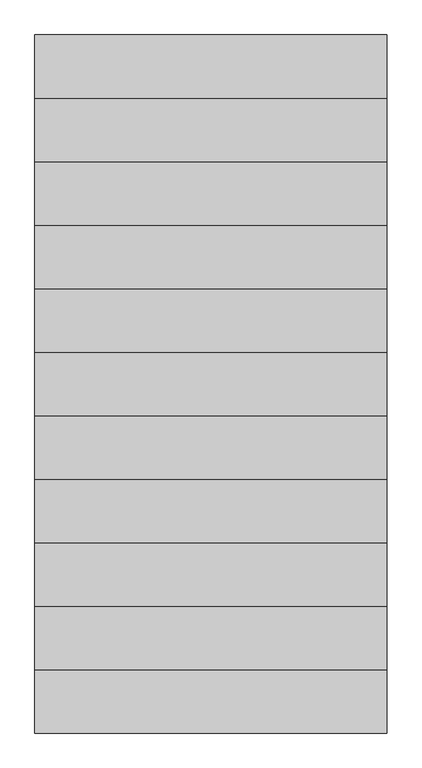
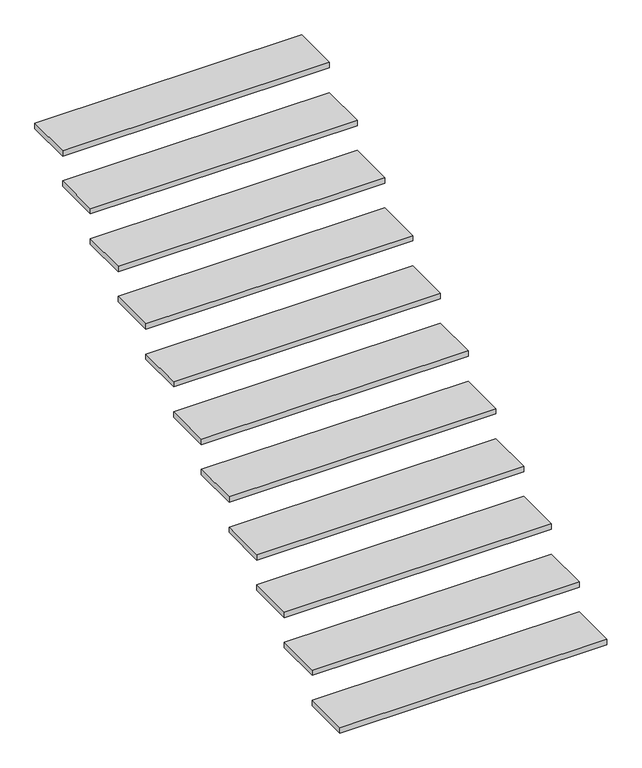
"""IFC4 building model written with IfcOpenShell, lengths in millimetres: stair flight geometry."""

from ifc_helpers import new_model, si_unit, frame, origin, place, context, project, spatial, polyline, outline, extrude, source, transform, mapped, element, save


def stair_flight_466a32d1(model_context):
    return source(origin(), model_context, "Body", "SweptSolid", [
        extrude(outline(polyline([(17005.3403387, 2217.6066446), (18505.3403387, 2217.6066446), (18505.3403387, 1947.6066446), (17005.3403387, 1947.6066446), (17005.3403387, 2217.6066446)])), frame((0.0, 0.0, 11969.0989011), z_axis=(0.0, 0.0, 1.0), x_axis=(1.0, 0.0, 0.0)), (0.0, 0.0, 1.0), 32.0),
        extrude(outline(polyline([(17005.3403387, 2487.6066446), (18505.3403387, 2487.6066446), (18505.3403387, 2217.6066446), (17005.3403387, 2217.6066446), (17005.3403387, 2487.6066446)])), frame((0.0, 0.0, 12148.2197802), z_axis=(0.0, 0.0, 1.0), x_axis=(1.0, 0.0, 0.0)), (0.0, 0.0, 1.0), 32.0),
        extrude(outline(polyline([(17005.3403387, 2757.6066446), (18505.3403387, 2757.6066446), (18505.3403387, 2487.6066446), (17005.3403387, 2487.6066446), (17005.3403387, 2757.6066446)])), frame((0.0, 0.0, 12327.3406593), z_axis=(0.0, 0.0, 1.0), x_axis=(1.0, 0.0, 0.0)), (0.0, 0.0, 1.0), 32.0),
        extrude(outline(polyline([(17005.3403387, 3027.6066446), (18505.3403387, 3027.6066446), (18505.3403387, 2757.6066446), (17005.3403387, 2757.6066446), (17005.3403387, 3027.6066446)])), frame((0.0, 0.0, 12506.4615385), z_axis=(0.0, 0.0, 1.0), x_axis=(1.0, 0.0, 0.0)), (0.0, 0.0, 1.0), 32.0),
        extrude(outline(polyline([(17005.3403387, 3297.6066446), (18505.3403387, 3297.6066446), (18505.3403387, 3027.6066446), (17005.3403387, 3027.6066446), (17005.3403387, 3297.6066446)])), frame((0.0, 0.0, 12685.5824176), z_axis=(0.0, 0.0, 1.0), x_axis=(1.0, 0.0, 0.0)), (0.0, 0.0, 1.0), 32.0),
        extrude(outline(polyline([(17005.3403387, 3567.6066446), (18505.3403387, 3567.6066446), (18505.3403387, 3297.6066446), (17005.3403387, 3297.6066446), (17005.3403387, 3567.6066446)])), frame((0.0, 0.0, 12864.7032967), z_axis=(0.0, 0.0, 1.0), x_axis=(1.0, 0.0, 0.0)), (0.0, 0.0, 1.0), 32.0),
        extrude(outline(polyline([(17005.3403387, 3837.6066446), (18505.3403387, 3837.6066446), (18505.3403387, 3567.6066446), (17005.3403387, 3567.6066446), (17005.3403387, 3837.6066446)])), frame((0.0, 0.0, 13043.8241758), z_axis=(0.0, 0.0, 1.0), x_axis=(1.0, 0.0, 0.0)), (0.0, 0.0, 1.0), 32.0),
        extrude(outline(polyline([(17005.3403387, 4107.6066446), (18505.3403387, 4107.6066446), (18505.3403387, 3837.6066446), (17005.3403387, 3837.6066446), (17005.3403387, 4107.6066446)])), frame((0.0, 0.0, 13222.9450549), z_axis=(0.0, 0.0, 1.0), x_axis=(1.0, 0.0, 0.0)), (0.0, 0.0, 1.0), 32.0),
        extrude(outline(polyline([(17005.3403387, 4377.6066446), (18505.3403387, 4377.6066446), (18505.3403387, 4107.6066446), (17005.3403387, 4107.6066446), (17005.3403387, 4377.6066446)])), frame((0.0, 0.0, 13402.0659341), z_axis=(0.0, 0.0, 1.0), x_axis=(1.0, 0.0, 0.0)), (0.0, 0.0, 1.0), 32.0),
        extrude(outline(polyline([(17005.3403387, 4647.6066446), (18505.3403387, 4647.6066446), (18505.3403387, 4377.6066446), (17005.3403387, 4377.6066446), (17005.3403387, 4647.6066446)])), frame((0.0, 0.0, 13581.1868132), z_axis=(0.0, 0.0, 1.0), x_axis=(1.0, 0.0, 0.0)), (0.0, 0.0, 1.0), 32.0),
        extrude(outline(polyline([(17005.3403387, 4917.6066446), (18505.3403387, 4917.6066446), (18505.3403387, 4647.6066446), (17005.3403387, 4647.6066446), (17005.3403387, 4917.6066446)])), frame((0.0, 0.0, 13760.3076923), z_axis=(0.0, 0.0, 1.0), x_axis=(1.0, 0.0, 0.0)), (0.0, 0.0, 1.0), 32.0),
    ])


if __name__ == "__main__":
    model = new_model("IFC4")
    model_context = context("Model", 3, world=origin())
    ifc_project = project(units=[si_unit("LENGTHUNIT", "METRE", prefix="MILLI")], contexts=[model_context])
    site = spatial("IfcSite", under=ifc_project)
    building = spatial("IfcBuilding", under=site)
    placement = place(None, origin())
    stair_flight_shape = stair_flight_466a32d1(model_context)
    element("IfcStairFlight", 1, at=placement, inside=building, context=model_context, shape_type="MappedRepresentation", body=[
        mapped(stair_flight_shape, transform((0.0, 0.0, 0.0), x_axis=(1.0, 0.0, 0.0), y_axis=(0.0, 1.0, 0.0), z_axis=(0.0, 0.0, 1.0))),
    ])
    save(model, "model.ifc")

# Revit data of these elements
# Element 1 (IfcStairFlight)
#   Materials on its faces: "철강"
# Materials
#   "철강": class "Generic", colour RGB 143 142 141, transparency 0, Description = "철골+가공조립+세우기", Cost = 0
